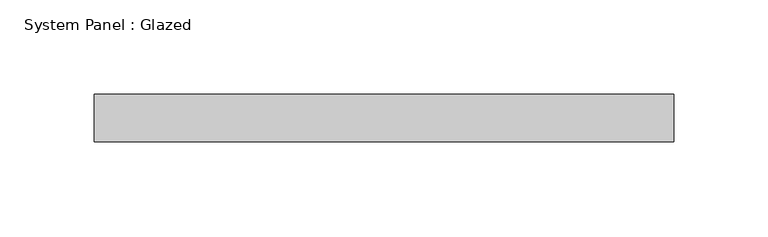
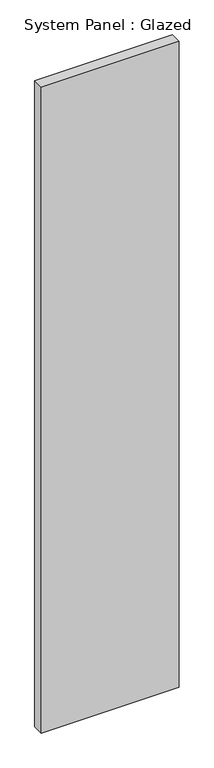
"""IFC4 building model written with IfcOpenShell, lengths in millimetres: plate geometry, System Panel : Glazed."""

from ifc_helpers import new_model, si_unit, origin, origin_with_axes, place, context, project, spatial, polyline, outline, extrude, source, transform, mapped, element, save


def system_panel_glazed_88f24eba(model_context):
    return source(origin(), model_context, "Body", "SweptSolid", [
        extrude(outline(polyline([(153.9999998, 19.05), (-153.9999998, 19.05), (-153.9999998, 44.45), (153.9999998, 44.45), (153.9999998, 19.05)])), origin_with_axes(), (0.0, 0.0, 1.0), 1524.0),
    ])


if __name__ == "__main__":
    model = new_model("IFC4")
    model_context = context("Model", 3, world=origin())
    ifc_project = project(units=[si_unit("LENGTHUNIT", "METRE", prefix="MILLI")], contexts=[model_context])
    site = spatial("IfcSite", under=ifc_project)
    building = spatial("IfcBuilding", under=site)
    placement = place(None, origin())
    system_panel_glazed_shape = system_panel_glazed_88f24eba(model_context)
    element("IfcPlate", 1, ObjectType="System Panel : Glazed", at=placement, inside=building, context=model_context, shape_type="MappedRepresentation", body=[
        mapped(system_panel_glazed_shape, transform((0.0, 0.0, 0.0), x_axis=(1.0, 0.0, 0.0), y_axis=(0.0, 1.0, 0.0), z_axis=(0.0, 0.0, 1.0))),
    ])
    save(model, "model.ifc")

# Revit data of these elements
# Type "System Panel : Glazed"
#   Construction Type Id = "GSP4R"
#   Analytic Construction = "1/8 in Pilkington single glazing"
#   Visual Light Transmittance = 0.9
#   Solar Heat Gain Coefficient = 0.86
#   Heat Transfer Coefficient (U) = 6.7069 W/(m²·K)
# Element 1 (IfcPlate, "System Panel : Glazed")
#   Materials on its faces: "Glass"
# Materials
#   "Glass": class "Glass", colour RGB 0 128 192, transparency 0.75, Description = "Soda Lime Glass", Cost = 0
